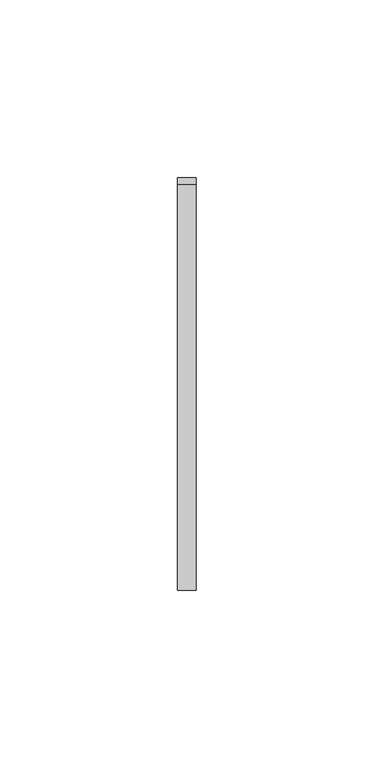
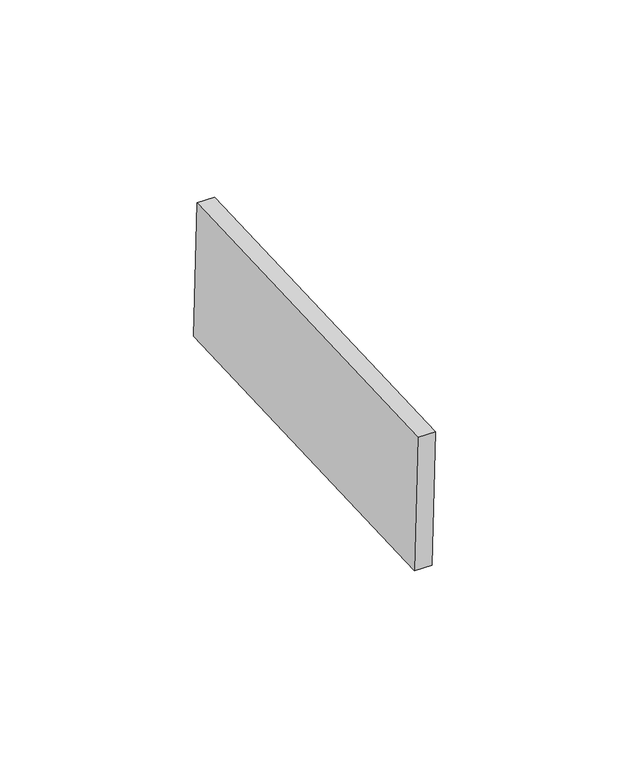
"""IFC4 building model written with IfcOpenShell, lengths in millimetres: proxy geometry, Inner panel:Inner panel:1:Inner panel:1 : Inner panel:Inner panel:300324:2:Inner panel:1:Inner panel:1 : Inner panel:Inner panel:300324:2 : Inner panel:Inner panel:1:Inner panel:1 : Inner panel:Inner panel:300324:300043:46 : Inner panel:Inner panel:1:Inner panel:1 : Inner panel:Inner panel:300324:2:Inner panel:1:Inner panel:1 : Inner panel:Inner panel:300324:2 : Inner panel:Inner panel:1:Inner panel:1 : Inner panel:Inner panel:300324:300043:308120."""

from ifc_helpers import new_model, si_unit, frame, origin, place, context, project, spatial, polyline, outline, extrude, source, transform, mapped, element, save


def generic_models_8a6294a4(model_context):
    return source(origin(), model_context, "Body", "SweptSolid", [
        extrude(outline(polyline([(0.0, -114.2999999), (0.0, 0.0), (5.2138089, 0.0), (5.2138089, -114.2999999), (0.0, -114.2999999)])), frame((593530.195117, -576618.8219505, 4051.6214343), z_axis=(0.0, -0.04163054471216399, 0.9991330730923527), x_axis=(-1.0, 0.0, 0.0)), (0.0, 0.0, 1.0), 43.2233908),
    ])


if __name__ == "__main__":
    model = new_model("IFC4")
    model_context = context("Model", 3, world=origin())
    ifc_project = project(units=[si_unit("LENGTHUNIT", "METRE", prefix="MILLI")], contexts=[model_context])
    site = spatial("IfcSite", under=ifc_project)
    building = spatial("IfcBuilding", under=site)
    placement = place(None, origin())
    generic_models_shape = generic_models_8a6294a4(model_context)
    element("IfcBuildingElementProxy", 1, Name="Inner panel:Inner panel:1:Inner panel:1 : Inner panel:Inner panel:300324:2:Inner panel:1:Inner panel:1 : Inner panel:Inner panel:300324:2 : Inner panel:Inner panel:1:Inner panel:1 : Inner panel:Inner panel:300324:300043:46 : Inner panel:Inner panel:1:Inner panel:1 : Inner panel:Inner panel:300324:2:Inner panel:1:Inner panel:1 : Inner panel:Inner panel:300324:2 : Inner panel:Inner panel:1:Inner panel:1 : Inner panel:Inner panel:300324:300043:308120", ObjectType="Inner panel:Inner panel:1:Inner panel:1 : Inner panel:Inner panel:300324:2:Inner panel:1:Inner panel:1 : Inner panel:Inner panel:300324:2 : Inner panel:Inner panel:1:Inner panel:1 : Inner panel:Inner panel:300324:300043:46 : Inner panel:Inner panel:1:Inner panel:1 : Inner panel:Inner panel:300324:2:Inner panel:1:Inner panel:1 : Inner panel:Inner panel:300324:2 : Inner panel:Inner panel:1:Inner panel:1 : Inner panel:Inner panel:300324:300043:308120", at=placement, inside=building, context=model_context, shape_type="MappedRepresentation", body=[
        mapped(generic_models_shape, transform((0.0, 0.0, 0.0), x_axis=(1.0, 0.0, 0.0), y_axis=(0.0, 1.0, 0.0), z_axis=(0.0, 0.0, 1.0))),
    ])
    save(model, "model.ifc")

# Revit data of these elements
# Type "Inner panel:Inner panel:1:Inner panel:1 : Inner panel:Inner panel:300324:2:Inner panel:1:Inner panel:1 : Inner panel:Inner panel:300324:2 : Inner panel:Inner panel:1:Inner panel:1 : Inner panel:Inner panel:300324:300043:46 : Inner panel:Inner panel:1:Inner panel:1 : Inner panel:Inner panel:300324:2:Inner panel:1:Inner panel:1 : Inner panel:Inner panel:300324:2 : Inner panel:Inner panel:1:Inner panel:1 : Inner panel:Inner panel:300324:300043:308120"
#   NameOverride = "Inner panel:Inner panel:1:Inner panel:1 : Inner panel:Inner panel:300324:2:Inner panel:1:Inner panel:1 : Inner panel:Inner panel:300324:2 : Inner panel:Inner panel:1:Inner panel:1 : Inner panel:Inner panel:300324:300043:308120"
#   ObjectTypeOverride = "Inner panel:1:Inner panel:1 : Inner panel:Inner panel:300324:2 : Inner panel:Inner panel:1:Inner panel:1 : Inner panel:Inner panel:300324:300043"
#   Reference = "Inner panel"
#   Tag = "308120"
# Element 1 (IfcBuildingElementProxy, "Inner panel:Inner panel:1:Inner panel:1 : Inner panel:Inner panel:300324:2:Inner panel:1:Inner panel:1 : Inner panel:Inner panel:300324:2 : Inner panel:Inner panel:1:Inner panel:1 : Inner panel:Inner panel:300324:300043:46 : Inner panel:Inner panel:1:Inner panel:1 : Inner panel:Inner panel:300324:2:Inner panel:1:Inner panel:1 : Inner panel:Inner panel:300324:2 : Inner panel:Inner panel:1:Inner panel:1 : Inner panel:Inner panel:300324:300043:308120")
#   Materials on its faces: "SLIDING CLIP"
# Materials
#   "SLIDING CLIP": class "Generic", colour RGB 120 120 120, transparency 0, Cost = 0
